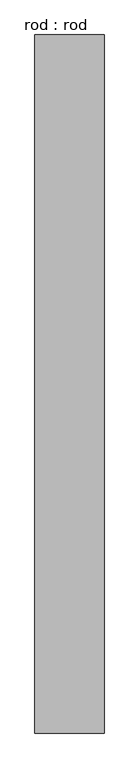
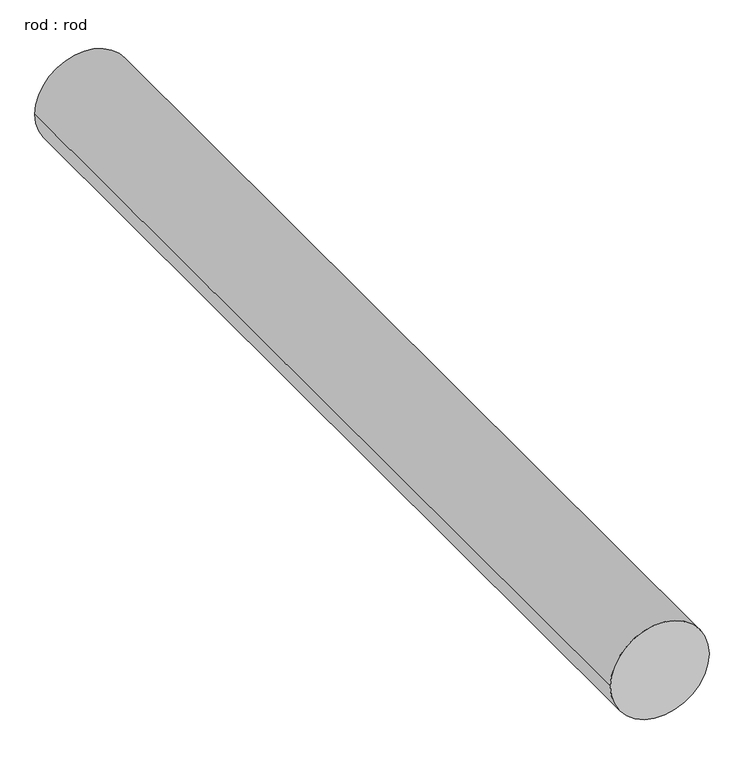
"""IFC4 building model written with IfcOpenShell, lengths in millimetres: proxy geometry, rod : rod."""

from ifc_helpers import new_model, si_unit, point, frame, frame_2d, origin, place, context, project, spatial, circle_curve, trimmed, segment, composite_curve, outline, extrude, source, transform, mapped, element, save


def rod_rod_76930b06(model_context):
    return source(origin(), model_context, "Body", "SweptSolid", [
        extrude(outline(composite_curve([segment(trimmed(circle_curve(frame_2d((0.0108462, 0.0)), 200.0), [point((0.0108462, 200.0))], [point((0.0108462, -200.0))], False, "CARTESIAN"), True, "CONTINUOUS"), segment(trimmed(circle_curve(frame_2d((0.0108462, 0.0)), 200.0), [point((0.0108462, -200.0))], [point((0.0108462, 200.0))], False, "CARTESIAN"), True, "CONTINUOUS")], self_intersect=False)), frame((0.0, 2072.4424351, 0.0), z_axis=(0.0, 1.0, 0.0), x_axis=(0.0, 0.0, 1.0)), (0.0, 0.0, 1.0), 4040.5723604),
    ])


if __name__ == "__main__":
    model = new_model("IFC4")
    model_context = context("Model", 3, world=origin())
    ifc_project = project(units=[si_unit("LENGTHUNIT", "METRE", prefix="MILLI")], contexts=[model_context])
    site = spatial("IfcSite", under=ifc_project)
    building = spatial("IfcBuilding", under=site)
    placement = place(None, origin())
    rod_rod_shape = rod_rod_76930b06(model_context)
    element("IfcBuildingElementProxy", 1, Name="rod : rod", ObjectType="rod : rod", at=placement, inside=building, context=model_context, shape_type="MappedRepresentation", body=[
        mapped(rod_rod_shape, transform((0.0, 0.0, 0.0), x_axis=(1.0, 0.0, 0.0), y_axis=(0.0, 1.0, 0.0), z_axis=(0.0, 0.0, 1.0))),
    ])
    save(model, "model.ifc")

# Revit data of these elements
# Type "rod : rod"
#   Default Elevation = 0
